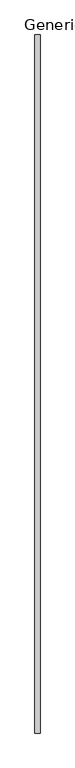
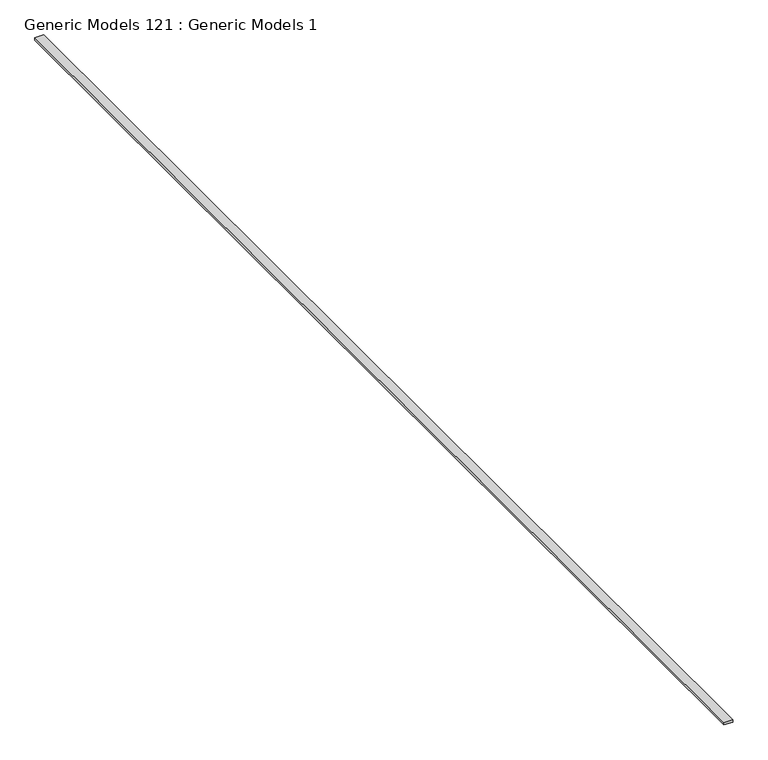
"""IFC4 building model written with IfcOpenShell, lengths in millimetres: proxy geometry, Generic Models 121 : Generic Models 1."""

from ifc_helpers import new_model, si_unit, frame, origin, place, context, project, spatial, polyline, outline, extrude, source, transform, mapped, element, save


def generic_models_121_generic_models_1_f60b4abb(model_context):
    return source(origin(), model_context, "Body", "SweptSolid", [
        extrude(outline(polyline([(7095.9513704, 11981.8769662), (7235.6513704, 11981.8769662), (7235.6513704, -7068.1230338), (7095.9513704, -7068.1230338), (7095.9513704, 11981.8769662)])), frame((0.0, 0.0, 127028.2735933), z_axis=(0.0, 0.0, 1.0), x_axis=(1.0, 0.0, 0.0)), (0.0, 0.0, 1.0), 38.1),
    ])


if __name__ == "__main__":
    model = new_model("IFC4")
    model_context = context("Model", 3, world=origin())
    ifc_project = project(units=[si_unit("LENGTHUNIT", "METRE", prefix="MILLI")], contexts=[model_context])
    site = spatial("IfcSite", under=ifc_project)
    building = spatial("IfcBuilding", under=site)
    placement = place(None, origin())
    generic_models_121_generic_models_1_shape = generic_models_121_generic_models_1_f60b4abb(model_context)
    element("IfcBuildingElementProxy", 1, Name="Generic Models 121 : Generic Models 1", ObjectType="Generic Models 121 : Generic Models 1", at=placement, inside=building, context=model_context, shape_type="MappedRepresentation", body=[
        mapped(generic_models_121_generic_models_1_shape, transform((0.0, 0.0, 0.0), x_axis=(1.0, 0.0, 0.0), y_axis=(0.0, 1.0, 0.0), z_axis=(0.0, 0.0, 1.0))),
    ])
    save(model, "model.ifc")

# Revit data of these elements
# Element 1 (IfcBuildingElementProxy, "Generic Models 121 : Generic Models 1")
#   Materials on its faces: "_2X BLOCKING AS REQUIRED"
# Materials
#   "_2X BLOCKING AS REQUIRED": class "Generic", colour RGB 177 130 114, transparency 0, Cost = 0
